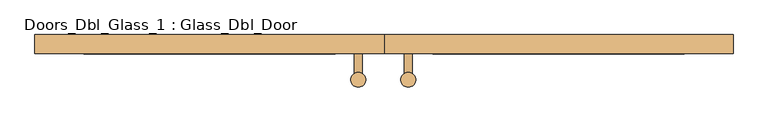
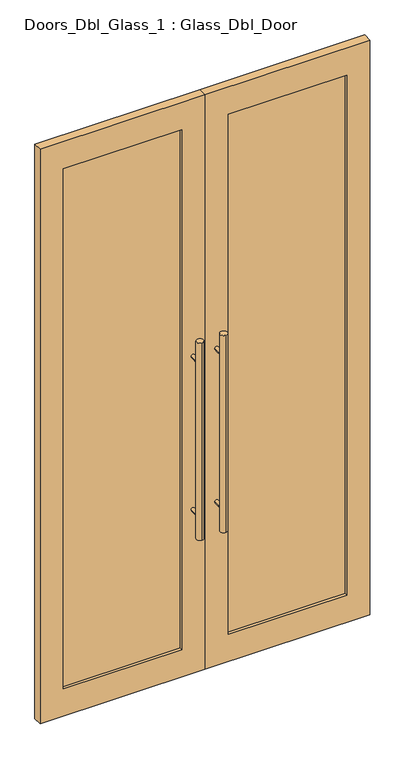
"""IFC4 building model written with IfcOpenShell, lengths in millimetres: door geometry, Doors_Dbl_Glass_1 : Glass_Dbl_Door."""

import ifcopenshell
import ifcopenshell.guid

model = None  # the IFC model being written
_history = None  # IfcOwnerHistory: only IFC2X3 demands one
_inside = {}  # id of a spatial element -> (the spatial element, [elements in it])
_under = {}  # id of a project, library or spatial element -> (it, [spatial elements below it])
_declared = {}  # id of a project -> (the project, [libraries it declares])
_typed = {}  # id of a type object -> (the type object, [elements of that type])
_made_of = {}  # id of a material, layer set ... -> (it, [elements and type objects made of it])


def new_model(schema):
    """Start an empty IFC model of exactly this schema.

    Asked for "IFC4X3", IfcOpenShell would pick the latest addendum, in which some entities
    have other attributes; the version numbers below select the first issue.
    IFC2X3 requires an IfcOwnerHistory on every rooted entity: one is made here for all.
    """
    global model, _history
    if schema == "IFC4X3":
        model = ifcopenshell.file(schema_version=(4, 3, 0, 0))
    else:
        model = ifcopenshell.file(schema=schema)
    _inside.clear()
    _under.clear()
    _declared.clear()
    _typed.clear()
    _made_of.clear()
    _history = None
    if model.schema == "IFC2X3":
        org = make("IfcOrganization", Name="unknown")
        user = make(
            "IfcPersonAndOrganization",
            ThePerson=make("IfcPerson", FamilyName="unknown"),
            TheOrganization=org,
        )
        app = make(
            "IfcApplication",
            ApplicationDeveloper=org,
            Version="unknown",
            ApplicationFullName="unknown",
            ApplicationIdentifier="unknown",
        )
        _history = make(
            "IfcOwnerHistory",
            OwningUser=user,
            OwningApplication=app,
            ChangeAction="ADDED",
            CreationDate=0,
        )
    return model


def make(cls, **values):
    """One entity of the class cls with the attributes given. An attribute that is None is left unset."""
    return model.create_entity(
        cls, **{name: value for name, value in values.items() if value is not None}
    )


def rooted(cls, **values):
    """An entity with a GlobalId (a new one), such as an element, a storey or a relation."""
    return make(cls, GlobalId=ifcopenshell.guid.new(), OwnerHistory=_history, **values)


def si_unit(unit_type, name, prefix=None):
    """IfcSIUnit, for example si_unit("LENGTHUNIT", "METRE", prefix="MILLI")."""
    return make("IfcSIUnit", UnitType=unit_type, Prefix=prefix, Name=name)


def assignment(units):
    """IfcUnitAssignment: the units of a project."""
    return None if units is None else make("IfcUnitAssignment", Units=units)


def point(xyz):
    """IfcCartesianPoint."""
    return None if xyz is None else make("IfcCartesianPoint", Coordinates=xyz)


def direction(xyz):
    """IfcDirection."""
    return None if xyz is None else make("IfcDirection", DirectionRatios=xyz)


def frame(location, z_axis=None, x_axis=None):
    """IfcAxis2Placement3D, a coordinate frame: its origin and axes. An axis left out is left unset."""
    return make(
        "IfcAxis2Placement3D",
        Location=point(location),
        Axis=direction(z_axis),
        RefDirection=direction(x_axis),
    )


def frame_2d(location, x_axis=None):
    """IfcAxis2Placement2D, a coordinate frame in the plane: its origin and x axis."""
    return make(
        "IfcAxis2Placement2D", Location=point(location), RefDirection=direction(x_axis)
    )


def origin():
    """The frame at (0, 0, 0) with its axes left unset."""
    return frame((0.0, 0.0, 0.0))


def place(relative_to, where):
    """IfcLocalPlacement: puts the frame where relative to a parent placement (None: the world)."""
    return make(
        "IfcLocalPlacement", PlacementRelTo=relative_to, RelativePlacement=where
    )


def context(
    kind, dimensions, precision=None, world=None, true_north=None, identifier=None
):
    """IfcGeometricRepresentationContext, for example the 3D "Model" context."""
    return make(
        "IfcGeometricRepresentationContext",
        ContextIdentifier=identifier,
        ContextType=kind,
        CoordinateSpaceDimension=dimensions,
        Precision=precision,
        WorldCoordinateSystem=world,
        TrueNorth=true_north,
    )


def project(units=None, contexts=None):
    """IfcProject with its units and contexts."""
    return rooted(
        "IfcProject",
        Name="project",
        RepresentationContexts=contexts,
        UnitsInContext=assignment(units),
    )


def spatial(cls, under=None, at=None, **own):
    """A site, building, storey or space (cls), placed at a placement, below another one or the project."""
    s = rooted(cls, ObjectPlacement=at, **own)
    if under is not None:
        _under.setdefault(under.id(), (under, []))[1].append(s)
    return s


def polyline(points):
    """IfcPolyline through the points."""
    return make("IfcPolyline", Points=[point(p) for p in points])


def circle_curve(where, radius):
    """IfcCircle in the frame where."""
    return make("IfcCircle", Position=where, Radius=radius)


def trimmed(basis, trim1, trim2, sense, master):
    """IfcTrimmedCurve: the piece of a basis curve between two trims."""
    return make(
        "IfcTrimmedCurve",
        BasisCurve=basis,
        Trim1=trim1,
        Trim2=trim2,
        SenseAgreement=sense,
        MasterRepresentation=master,
    )


def segment(curve, same_sense, transition):
    """IfcCompositeCurveSegment."""
    return make(
        "IfcCompositeCurveSegment",
        Transition=transition,
        SameSense=same_sense,
        ParentCurve=curve,
    )


def composite_curve(segments, self_intersect=None):
    """IfcCompositeCurve: segments joined end to end."""
    return make("IfcCompositeCurve", Segments=segments, SelfIntersect=self_intersect)


def outline(outer, holes=None, kind="AREA"):
    """IfcArbitraryClosedProfileDef: a profile drawn as a closed curve; with holes, ...WithVoids."""
    if holes is None:
        return make("IfcArbitraryClosedProfileDef", ProfileType=kind, OuterCurve=outer)
    return make(
        "IfcArbitraryProfileDefWithVoids",
        ProfileType=kind,
        OuterCurve=outer,
        InnerCurves=holes,
    )


def extrude(swept, where, along, depth):
    """IfcExtrudedAreaSolid: the profile swept, set in the frame where, extruded along a direction by depth."""
    return make(
        "IfcExtrudedAreaSolid",
        SweptArea=swept,
        Position=where,
        ExtrudedDirection=direction(along),
        Depth=depth,
    )


def shape(context_of_items, identifier, shape_type, items):
    """IfcShapeRepresentation: the items that make up one representation, for example the "Body"."""
    return make(
        "IfcShapeRepresentation",
        ContextOfItems=context_of_items,
        RepresentationIdentifier=identifier,
        RepresentationType=shape_type,
        Items=items,
    )


def source(mapping_origin, context_of_items, identifier, shape_type, items):
    """IfcRepresentationMap: a shape defined once, which mapped items show again and again."""
    return make(
        "IfcRepresentationMap",
        MappingOrigin=mapping_origin,
        MappedRepresentation=shape(context_of_items, identifier, shape_type, items),
    )


def transform(
    local_origin,
    x_axis=None,
    y_axis=None,
    z_axis=None,
    scale=None,
    scale2=None,
    scale3=None,
    uniform=True,
):
    """IfcCartesianTransformationOperator3D, or its non-uniform kind. x_axis, y_axis, z_axis: its Axis1, 2, 3."""
    if uniform:
        return make(
            "IfcCartesianTransformationOperator3D",
            Axis1=direction(x_axis),
            Axis2=direction(y_axis),
            LocalOrigin=point(local_origin),
            Scale=scale,
            Axis3=direction(z_axis),
        )
    return make(
        "IfcCartesianTransformationOperator3DnonUniform",
        Axis1=direction(x_axis),
        Axis2=direction(y_axis),
        LocalOrigin=point(local_origin),
        Scale=scale,
        Axis3=direction(z_axis),
        Scale2=scale2,
        Scale3=scale3,
    )


def mapped(mapping_source, mapping_target):
    """IfcMappedItem: shows the shape of a source again, moved by a transform."""
    return make(
        "IfcMappedItem", MappingSource=mapping_source, MappingTarget=mapping_target
    )


def made_of(thing, what):
    """Note that an element or type object is made of a material, layer set ...; save() writes the relation."""
    if what is not None:
        _made_of.setdefault(what.id(), (what, []))[1].append(thing)
    return thing


def element(
    cls,
    number,
    at=None,
    inside=None,
    cuts=None,
    type_object=None,
    material=None,
    context=None,
    identifier="Body",
    shape_type=None,
    held_by="IfcProductDefinitionShape",
    body=None,
    shapes=None,
    **own,
):
    """One element of the class cls, such as IfcWall. Its Tag is "e" and its number.

    at: its placement. inside: the storey or other place that contains it. cuts: it is an
    opening in that element (IfcRelVoidsElement). A single representation is given by context,
    identifier, shape_type and body (its items); several are given by shapes. held_by: the class
    of the entity that holds the representations. save() writes the other relations.
    """
    e = rooted(cls, Tag="e%d" % number, ObjectPlacement=at, **own)
    if body is not None:
        shapes = [shape(context, identifier, shape_type, body)]
    if shapes is not None:
        e.Representation = make(held_by, Representations=shapes)
    if inside is not None:
        _inside.setdefault(inside.id(), (inside, []))[1].append(e)
    if cuts is not None:
        rooted(
            "IfcRelVoidsElement", RelatingBuildingElement=cuts, RelatedOpeningElement=e
        )
    if type_object is not None:
        _typed.setdefault(type_object.id(), (type_object, []))[1].append(e)
    return made_of(e, material)


def aggregate(whole, parts):
    """IfcRelAggregates: a whole, such as a stair, and the parts it consists of."""
    return rooted("IfcRelAggregates", RelatingObject=whole, RelatedObjects=parts)


def save(model, path):
    """Write the relations noted so far, then the file.

    IfcRelAggregates (storeys below a building ...), IfcRelContainedInSpatialStructure (elements
    in a storey), IfcRelDefinesByType, IfcRelAssociatesMaterial and IfcRelDeclares: one each for
    every whole, place, type object, material and project.
    """
    for whole, parts in _under.values():
        aggregate(whole, parts)
    for where, things in _inside.values():
        rooted(
            "IfcRelContainedInSpatialStructure",
            RelatedElements=things,
            RelatingStructure=where,
        )
    for kind, things in _typed.values():
        rooted("IfcRelDefinesByType", RelatedObjects=things, RelatingType=kind)
    for what, things in _made_of.values():
        rooted("IfcRelAssociatesMaterial", RelatedObjects=things, RelatingMaterial=what)
    for by, libraries in _declared.values():
        rooted("IfcRelDeclares", RelatingContext=by, RelatedDefinitions=libraries)
    model.write(path)


def doors_dbl_glass_1_glass_dbl_door_233ab62a(model_context):
    return source(origin(), model_context, "Body", "SweptSolid", [
        extrude(outline(composite_curve([segment(trimmed(circle_curve(frame_2d((49.6069979, -116.0715804)), 15.0), [point((49.6069979, -101.0715804))], [point((49.6069979, -131.0715804))], False, "CARTESIAN"), True, "CONTINUOUS"), segment(trimmed(circle_curve(frame_2d((49.6069979, -116.0715804)), 15.0), [point((49.6069979, -131.0715804))], [point((49.6069979, -101.0715804))], False, "CARTESIAN"), True, "CONTINUOUS")], self_intersect=False)), frame((0.0, 0.0, 650.0), z_axis=(0.0, 0.0, 1.0), x_axis=(1.0, 0.0, 0.0)), (0.0, 0.0, 1.0), 900.0),
        extrude(outline(composite_curve([segment(trimmed(circle_curve(frame_2d((-52.537897, -116.0715804)), 15.0), [point((-52.537897, -101.0715804))], [point((-52.537897, -131.0715804))], False, "CARTESIAN"), True, "CONTINUOUS"), segment(trimmed(circle_curve(frame_2d((-52.537897, -116.0715804)), 15.0), [point((-52.537897, -131.0715804))], [point((-52.537897, -101.0715804))], False, "CARTESIAN"), True, "CONTINUOUS")], self_intersect=False)), frame((0.0, 0.0, 650.0), z_axis=(0.0, 0.0, 1.0), x_axis=(1.0, 0.0, 0.0)), (0.0, 0.0, 1.0), 900.0),
        extrude(outline(composite_curve([segment(trimmed(circle_curve(frame_2d((750.0, 49.6069979)), 8.0), [point((750.0, 57.6069979))], [point((750.0, 41.6069979))], False, "CARTESIAN"), True, "CONTINUOUS"), segment(trimmed(circle_curve(frame_2d((750.0, 49.6069979)), 8.0), [point((750.0, 41.6069979))], [point((750.0, 57.6069979))], False, "CARTESIAN"), True, "CONTINUOUS")], self_intersect=False)), frame((0.0, -116.0715804, 0.0), z_axis=(0.0, 1.0, 0.0), x_axis=(0.0, 0.0, 1.0)), (0.0, 0.0, 1.0), 53.4927248),
        extrude(outline(composite_curve([segment(trimmed(circle_curve(frame_2d((750.0, -52.537897)), 8.0), [point((750.0, -44.537897))], [point((750.0, -60.537897))], False, "CARTESIAN"), True, "CONTINUOUS"), segment(trimmed(circle_curve(frame_2d((750.0, -52.537897)), 8.0), [point((750.0, -60.537897))], [point((750.0, -44.537897))], False, "CARTESIAN"), True, "CONTINUOUS")], self_intersect=False)), frame((0.0, -116.0715804, 0.0), z_axis=(0.0, 1.0, 0.0), x_axis=(0.0, 0.0, 1.0)), (0.0, 0.0, 1.0), 53.4927248),
        extrude(outline(composite_curve([segment(trimmed(circle_curve(frame_2d((1450.0, 49.6069979)), 8.0), [point((1450.0, 57.6069979))], [point((1450.0, 41.6069979))], False, "CARTESIAN"), True, "CONTINUOUS"), segment(trimmed(circle_curve(frame_2d((1450.0, 49.6069979)), 8.0), [point((1450.0, 41.6069979))], [point((1450.0, 57.6069979))], False, "CARTESIAN"), True, "CONTINUOUS")], self_intersect=False)), frame((0.0, -116.0715804, 0.0), z_axis=(0.0, 1.0, 0.0), x_axis=(0.0, 0.0, 1.0)), (0.0, 0.0, 1.0), 53.4927248),
        extrude(outline(composite_curve([segment(trimmed(circle_curve(frame_2d((1450.0, -52.537897)), 8.0), [point((1450.0, -44.537897))], [point((1450.0, -60.537897))], False, "CARTESIAN"), True, "CONTINUOUS"), segment(trimmed(circle_curve(frame_2d((1450.0, -52.537897)), 8.0), [point((1450.0, -60.537897))], [point((1450.0, -44.537897))], False, "CARTESIAN"), True, "CONTINUOUS")], self_intersect=False)), frame((0.0, -116.0715804, 0.0), z_axis=(0.0, 1.0, 0.0), x_axis=(0.0, 0.0, 1.0)), (0.0, 0.0, 1.0), 53.4927248),
        extrude(outline(polyline([(2625.0, -712.5), (0.0, -712.5), (0.0, 0.0), (2625.0, 0.0), (2625.0, -712.5)]), holes=[polyline([(2500.0, -612.5), (2500.0, -100.0), (125.0, -100.0), (125.0, -612.5), (2500.0, -612.5)])]), frame((0.0, -62.5788556, 0.0), z_axis=(0.0, 1.0, 0.0), x_axis=(0.0, 0.0, 1.0)), (0.0, 0.0, 1.0), 38.5435966),
        extrude(outline(polyline([(2625.0, 0.0), (0.0, 0.0), (0.0, 712.5), (2625.0, 712.5), (2625.0, 0.0)]), holes=[polyline([(2500.0, 100.0), (2500.0, 612.5), (125.0, 612.5), (125.0, 100.0), (2500.0, 100.0)])]), frame((0.0, -62.5788556, 0.0), z_axis=(0.0, 1.0, 0.0), x_axis=(0.0, 0.0, 1.0)), (0.0, 0.0, 1.0), 38.5435966),
        extrude(outline(polyline([(-100.0, -38.0), (-100.0, -50.0), (-612.5, -50.0), (-612.5, -38.0), (-100.0, -38.0)])), frame((0.0, 0.0, 125.0), z_axis=(0.0, 0.0, 1.0), x_axis=(1.0, 0.0, 0.0)), (0.0, 0.0, 1.0), 2375.0),
        extrude(outline(polyline([(612.5, -38.0), (612.5, -50.0), (100.0, -50.0), (100.0, -38.0), (612.5, -38.0)])), frame((0.0, 0.0, 125.0), z_axis=(0.0, 0.0, 1.0), x_axis=(1.0, 0.0, 0.0)), (0.0, 0.0, 1.0), 2375.0),
    ])


if __name__ == "__main__":
    model = new_model("IFC4")
    model_context = context("Model", 3, world=origin())
    ifc_project = project(units=[si_unit("LENGTHUNIT", "METRE", prefix="MILLI")], contexts=[model_context])
    site = spatial("IfcSite", under=ifc_project)
    building = spatial("IfcBuilding", under=site)
    placement = place(None, origin())
    doors_dbl_glass_1_glass_dbl_door_shape = doors_dbl_glass_1_glass_dbl_door_233ab62a(model_context)
    element("IfcDoor", 1, ObjectType="Doors_Dbl_Glass_1 : Glass_Dbl_Door", at=placement, inside=building, context=model_context, shape_type="MappedRepresentation", body=[
        mapped(doors_dbl_glass_1_glass_dbl_door_shape, transform((0.0, 0.0, 0.0), x_axis=(1.0, 0.0, 0.0), y_axis=(0.0, 1.0, 0.0), z_axis=(0.0, 0.0, 1.0))),
    ])
    save(model, "model.ifc")

# Revit data of these elements
# Project information
#   Project Issue Date = "Issue Date"
#   Project Status = "Project Status"
#   Client Name = "Owner"
#   Project Address = "Enter address here"
#   Project Name = "Project Name"
#   Project Number = "Project Number"
# Type "Doors_Dbl_Glass_1 : Glass_Dbl_Door"
#   Type Mark = "48"
#   Construction Type Id = "GSP4R"
#   Analytic Construction = "1/8 in Pilkington single glazing"
#   Visual Light Transmittance = 0.9
#   Stile Shutting = 100 mm
#   Stile Hanging = 100 mm
#   Stile - Top Rail = 125 mm
#   Stile - Bottom Rail = 125 mm
#   Solar Heat Gain Coefficient = 0.78
#   Offset = 50 mm
#   Heat Transfer Coefficient (U) = 3.6886 W/(m²·K)
#   Glass Thickness = 12 mm
#   Material Ironmongery = Metal - Aluminum
#   Material Door = Metal - Aluminum
#   Material Glass = Glass
#   Function = (empty or 0)
# Element 1 (IfcDoor, "Doors_Dbl_Glass_1 : Glass_Dbl_Door")
#   Materials on its faces: "Metal - Aluminum", "Glass"
# Materials
#   "Metal - Aluminum": class "Metal", colour RGB 247 247 247, transparency 0
#   "Glass": class "Glass", colour RGB 0 128 192, transparency 0.9, Description = "Soda Lime Glass", Cost = 0
